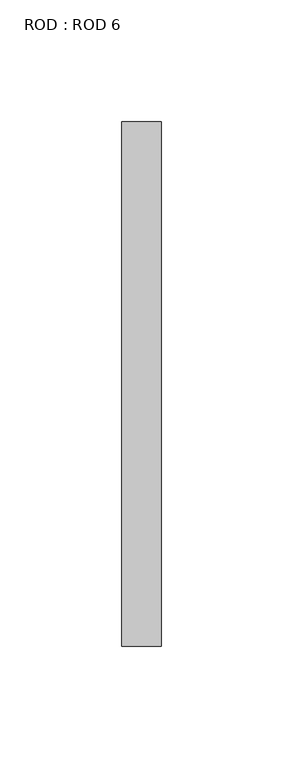
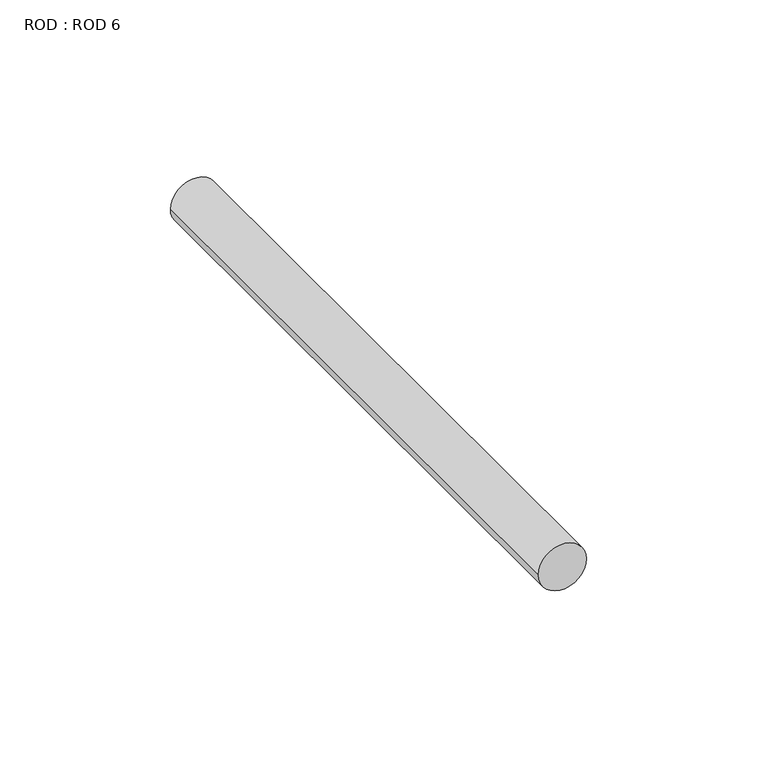
"""IFC4 building model written with IfcOpenShell, lengths in millimetres: proxy geometry, ROD : ROD 6."""

from ifc_helpers import new_model, si_unit, point, frame, origin, origin_2d, place, context, project, spatial, circle_curve, trimmed, segment, composite_curve, outline, extrude, source, transform, mapped, element, save


def rod_rod_6_b665ae48(model_context):
    return source(origin(), model_context, "Body", "SweptSolid", [
        extrude(outline(composite_curve([segment(trimmed(circle_curve(origin_2d(), 8.1359375), [point((0.0, 8.1359375))], [point((0.0, -8.1359375))], False, "CARTESIAN"), True, "CONTINUOUS"), segment(trimmed(circle_curve(origin_2d(), 8.1359375), [point((0.0, -8.1359375))], [point((0.0, 8.1359375))], False, "CARTESIAN"), True, "CONTINUOUS")], self_intersect=False)), frame((0.0, -152.4, 0.0), z_axis=(0.0, 1.0, 0.0), x_axis=(0.0, 0.0, 1.0)), (0.0, 0.0, 1.0), 215.9),
    ])


if __name__ == "__main__":
    model = new_model("IFC4")
    model_context = context("Model", 3, world=origin())
    ifc_project = project(units=[si_unit("LENGTHUNIT", "METRE", prefix="MILLI")], contexts=[model_context])
    site = spatial("IfcSite", under=ifc_project)
    building = spatial("IfcBuilding", under=site)
    placement = place(None, origin())
    rod_rod_6_shape = rod_rod_6_b665ae48(model_context)
    element("IfcBuildingElementProxy", 1, Name="ROD : ROD 6", ObjectType="ROD : ROD 6", at=placement, inside=building, context=model_context, shape_type="MappedRepresentation", body=[
        mapped(rod_rod_6_shape, transform((0.0, 0.0, 0.0), x_axis=(1.0, 0.0, 0.0), y_axis=(0.0, 1.0, 0.0), z_axis=(0.0, 0.0, 1.0))),
    ])
    save(model, "model.ifc")

# Revit data of these elements
# Type "ROD : ROD 6"
#   lenght = 0' - 8 1/2"
#   Radius = 0' - 0 41/128"
#   material [instance default] = 3/4" GALV. THRU BOLTS
# Materials
#   "3/4\" GALV. THRU BOLTS": class "Generic", colour RGB 105 69 171, transparency 0, Cost = 0
